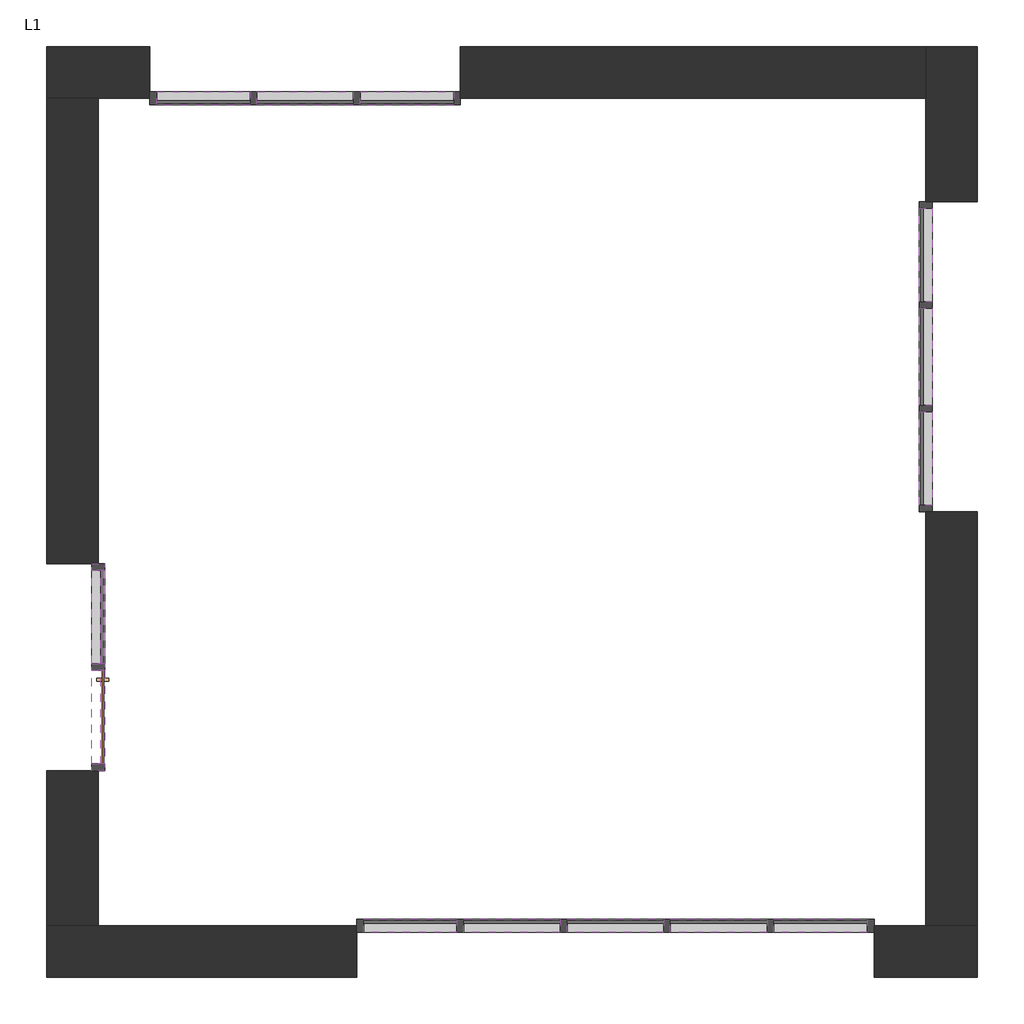
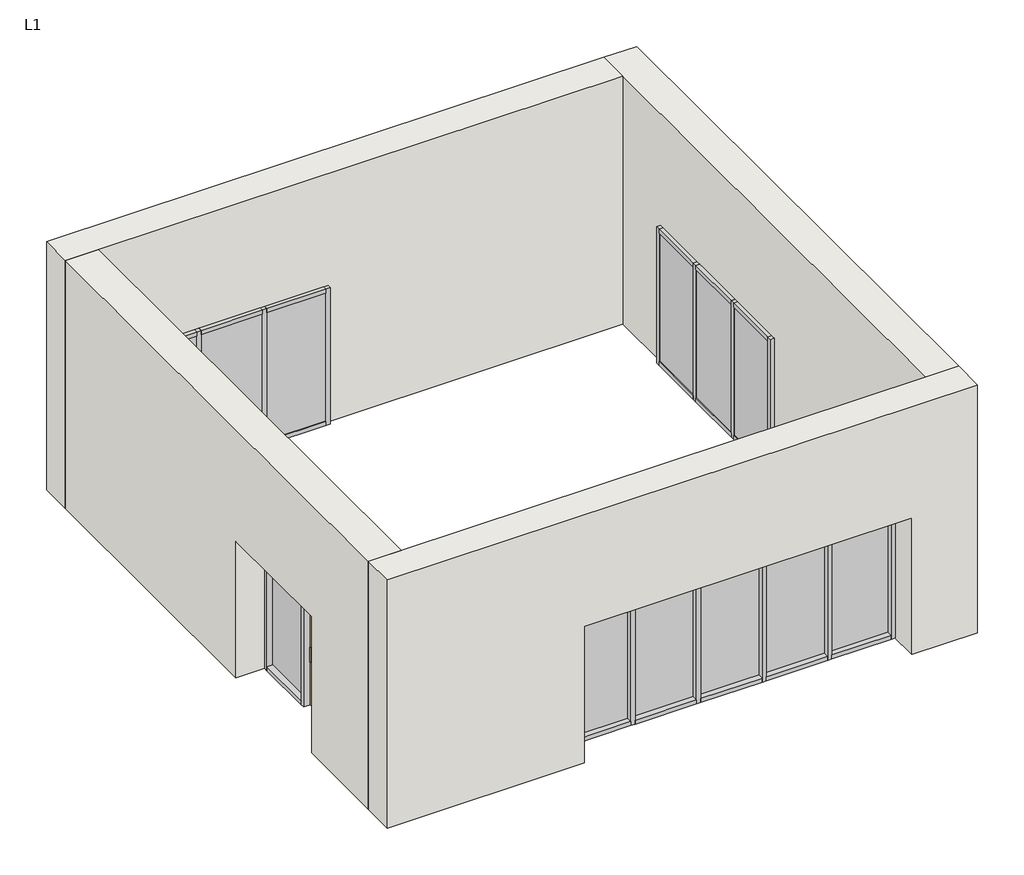
# One storey: 47 members, 14 plates, 4 walls, 1 door.
"""IFC4 building model written with IfcOpenShell, lengths in millimetres."""

import ifcopenshell
import ifcopenshell.guid

model = None  # the IFC model being written
_history = None  # IfcOwnerHistory: only IFC2X3 demands one
_inside = {}  # id of a spatial element -> (the spatial element, [elements in it])
_under = {}  # id of a project, library or spatial element -> (it, [spatial elements below it])
_declared = {}  # id of a project -> (the project, [libraries it declares])
_typed = {}  # id of a type object -> (the type object, [elements of that type])
_made_of = {}  # id of a material, layer set ... -> (it, [elements and type objects made of it])


def new_model(schema):
    """Start an empty IFC model of exactly this schema.

    Asked for "IFC4X3", IfcOpenShell would pick the latest addendum, in which some entities
    have other attributes; the version numbers below select the first issue.
    IFC2X3 requires an IfcOwnerHistory on every rooted entity: one is made here for all.
    """
    global model, _history
    if schema == "IFC4X3":
        model = ifcopenshell.file(schema_version=(4, 3, 0, 0))
    else:
        model = ifcopenshell.file(schema=schema)
    _inside.clear()
    _under.clear()
    _declared.clear()
    _typed.clear()
    _made_of.clear()
    _history = None
    if model.schema == "IFC2X3":
        org = make("IfcOrganization", Name="unknown")
        user = make(
            "IfcPersonAndOrganization",
            ThePerson=make("IfcPerson", FamilyName="unknown"),
            TheOrganization=org,
        )
        app = make(
            "IfcApplication",
            ApplicationDeveloper=org,
            Version="unknown",
            ApplicationFullName="unknown",
            ApplicationIdentifier="unknown",
        )
        _history = make(
            "IfcOwnerHistory",
            OwningUser=user,
            OwningApplication=app,
            ChangeAction="ADDED",
            CreationDate=0,
        )
    return model


def make(cls, **values):
    """One entity of the class cls with the attributes given. An attribute that is None is left unset."""
    return model.create_entity(
        cls, **{name: value for name, value in values.items() if value is not None}
    )


def rooted(cls, **values):
    """An entity with a GlobalId (a new one), such as an element, a storey or a relation."""
    return make(cls, GlobalId=ifcopenshell.guid.new(), OwnerHistory=_history, **values)


def si_unit(unit_type, name, prefix=None):
    """IfcSIUnit, for example si_unit("LENGTHUNIT", "METRE", prefix="MILLI")."""
    return make("IfcSIUnit", UnitType=unit_type, Prefix=prefix, Name=name)


def assignment(units):
    """IfcUnitAssignment: the units of a project."""
    return None if units is None else make("IfcUnitAssignment", Units=units)


def point(xyz):
    """IfcCartesianPoint."""
    return None if xyz is None else make("IfcCartesianPoint", Coordinates=xyz)


def direction(xyz):
    """IfcDirection."""
    return None if xyz is None else make("IfcDirection", DirectionRatios=xyz)


def frame(location, z_axis=None, x_axis=None):
    """IfcAxis2Placement3D, a coordinate frame: its origin and axes. An axis left out is left unset."""
    return make(
        "IfcAxis2Placement3D",
        Location=point(location),
        Axis=direction(z_axis),
        RefDirection=direction(x_axis),
    )


def origin():
    """The frame at (0, 0, 0) with its axes left unset."""
    return frame((0.0, 0.0, 0.0))


def origin_with_axes():
    """The frame at (0, 0, 0) with the z axis (0, 0, 1) and the x axis (1, 0, 0) written out."""
    return frame((0.0, 0.0, 0.0), z_axis=(0.0, 0.0, 1.0), x_axis=(1.0, 0.0, 0.0))


def place(relative_to, where):
    """IfcLocalPlacement: puts the frame where relative to a parent placement (None: the world)."""
    return make(
        "IfcLocalPlacement", PlacementRelTo=relative_to, RelativePlacement=where
    )


def context(
    kind, dimensions, precision=None, world=None, true_north=None, identifier=None
):
    """IfcGeometricRepresentationContext, for example the 3D "Model" context."""
    return make(
        "IfcGeometricRepresentationContext",
        ContextIdentifier=identifier,
        ContextType=kind,
        CoordinateSpaceDimension=dimensions,
        Precision=precision,
        WorldCoordinateSystem=world,
        TrueNorth=true_north,
    )


def project(units=None, contexts=None):
    """IfcProject with its units and contexts."""
    return rooted(
        "IfcProject",
        Name="project",
        RepresentationContexts=contexts,
        UnitsInContext=assignment(units),
    )


def spatial(cls, under=None, at=None, **own):
    """A site, building, storey or space (cls), placed at a placement, below another one or the project."""
    s = rooted(cls, ObjectPlacement=at, **own)
    if under is not None:
        _under.setdefault(under.id(), (under, []))[1].append(s)
    return s


def polyline(points):
    """IfcPolyline through the points."""
    return make("IfcPolyline", Points=[point(p) for p in points])


def outline(outer, holes=None, kind="AREA"):
    """IfcArbitraryClosedProfileDef: a profile drawn as a closed curve; with holes, ...WithVoids."""
    if holes is None:
        return make("IfcArbitraryClosedProfileDef", ProfileType=kind, OuterCurve=outer)
    return make(
        "IfcArbitraryProfileDefWithVoids",
        ProfileType=kind,
        OuterCurve=outer,
        InnerCurves=holes,
    )


def extrude(swept, where, along, depth):
    """IfcExtrudedAreaSolid: the profile swept, set in the frame where, extruded along a direction by depth."""
    return make(
        "IfcExtrudedAreaSolid",
        SweptArea=swept,
        Position=where,
        ExtrudedDirection=direction(along),
        Depth=depth,
    )


def faces_of(points, faces, orient=None, outer=None):
    """IfcFace entities. A face is a list of loops; a loop is a list of indices into points, from 0.

    orient and outer hold one flag for each loop. By default every Orientation is true, the
    first loop of a face is its IfcFaceOuterBound and the others are IfcFaceBound.
    """
    made = []
    for i, loops in enumerate(faces):
        bounds = []
        for j, loop in enumerate(loops):
            is_outer = j == 0 if outer is None else outer[i][j]
            bounds.append(
                make(
                    "IfcFaceOuterBound" if is_outer else "IfcFaceBound",
                    Bound=make("IfcPolyLoop", Polygon=[points[k] for k in loop]),
                    Orientation=True if orient is None else orient[i][j],
                )
            )
        made.append(make("IfcFace", Bounds=bounds))
    return made


def faceted_brep(points, faces, orient=None, outer=None, voids=None):
    """IfcFacetedBrep: a solid bounded by flat faces; with voids (closed shells), ...WithVoids."""
    shared = [point(p) for p in points]
    hull = make("IfcClosedShell", CfsFaces=faces_of(shared, faces, orient, outer))
    if voids is None:
        return make("IfcFacetedBrep", Outer=hull)
    return make(
        "IfcFacetedBrepWithVoids",
        Outer=hull,
        Voids=[
            make(cls, CfsFaces=faces_of(shared, fs, o, b)) for cls, fs, o, b in voids
        ],
    )


def shape(context_of_items, identifier, shape_type, items):
    """IfcShapeRepresentation: the items that make up one representation, for example the "Body"."""
    return make(
        "IfcShapeRepresentation",
        ContextOfItems=context_of_items,
        RepresentationIdentifier=identifier,
        RepresentationType=shape_type,
        Items=items,
    )


def source(mapping_origin, context_of_items, identifier, shape_type, items):
    """IfcRepresentationMap: a shape defined once, which mapped items show again and again."""
    return make(
        "IfcRepresentationMap",
        MappingOrigin=mapping_origin,
        MappedRepresentation=shape(context_of_items, identifier, shape_type, items),
    )


def transform(
    local_origin,
    x_axis=None,
    y_axis=None,
    z_axis=None,
    scale=None,
    scale2=None,
    scale3=None,
    uniform=True,
):
    """IfcCartesianTransformationOperator3D, or its non-uniform kind. x_axis, y_axis, z_axis: its Axis1, 2, 3."""
    if uniform:
        return make(
            "IfcCartesianTransformationOperator3D",
            Axis1=direction(x_axis),
            Axis2=direction(y_axis),
            LocalOrigin=point(local_origin),
            Scale=scale,
            Axis3=direction(z_axis),
        )
    return make(
        "IfcCartesianTransformationOperator3DnonUniform",
        Axis1=direction(x_axis),
        Axis2=direction(y_axis),
        LocalOrigin=point(local_origin),
        Scale=scale,
        Axis3=direction(z_axis),
        Scale2=scale2,
        Scale3=scale3,
    )


def mapped(mapping_source, mapping_target):
    """IfcMappedItem: shows the shape of a source again, moved by a transform."""
    return make(
        "IfcMappedItem", MappingSource=mapping_source, MappingTarget=mapping_target
    )


def made_of(thing, what):
    """Note that an element or type object is made of a material, layer set ...; save() writes the relation."""
    if what is not None:
        _made_of.setdefault(what.id(), (what, []))[1].append(thing)
    return thing


def element(
    cls,
    number,
    at=None,
    inside=None,
    cuts=None,
    type_object=None,
    material=None,
    context=None,
    identifier="Body",
    shape_type=None,
    held_by="IfcProductDefinitionShape",
    body=None,
    shapes=None,
    **own,
):
    """One element of the class cls, such as IfcWall. Its Tag is "e" and its number.

    at: its placement. inside: the storey or other place that contains it. cuts: it is an
    opening in that element (IfcRelVoidsElement). A single representation is given by context,
    identifier, shape_type and body (its items); several are given by shapes. held_by: the class
    of the entity that holds the representations. save() writes the other relations.
    """
    e = rooted(cls, Tag="e%d" % number, ObjectPlacement=at, **own)
    if body is not None:
        shapes = [shape(context, identifier, shape_type, body)]
    if shapes is not None:
        e.Representation = make(held_by, Representations=shapes)
    if inside is not None:
        _inside.setdefault(inside.id(), (inside, []))[1].append(e)
    if cuts is not None:
        rooted(
            "IfcRelVoidsElement", RelatingBuildingElement=cuts, RelatedOpeningElement=e
        )
    if type_object is not None:
        _typed.setdefault(type_object.id(), (type_object, []))[1].append(e)
    return made_of(e, material)


def aggregate(whole, parts):
    """IfcRelAggregates: a whole, such as a stair, and the parts it consists of."""
    return rooted("IfcRelAggregates", RelatingObject=whole, RelatedObjects=parts)


def save(model, path):
    """Write the relations noted so far, then the file.

    IfcRelAggregates (storeys below a building ...), IfcRelContainedInSpatialStructure (elements
    in a storey), IfcRelDefinesByType, IfcRelAssociatesMaterial and IfcRelDeclares: one each for
    every whole, place, type object, material and project.
    """
    for whole, parts in _under.values():
        aggregate(whole, parts)
    for where, things in _inside.values():
        rooted(
            "IfcRelContainedInSpatialStructure",
            RelatedElements=things,
            RelatingStructure=where,
        )
    for kind, things in _typed.values():
        rooted("IfcRelDefinesByType", RelatedObjects=things, RelatingType=kind)
    for what, things in _made_of.values():
        rooted("IfcRelAssociatesMaterial", RelatedObjects=things, RelatingMaterial=what)
    for by, libraries in _declared.values():
        rooted("IfcRelDeclares", RelatingContext=by, RelatedDefinitions=libraries)
    model.write(path)


def m_door_curtain_wall_single_glass_m_door_curtain_wall_single_b3f25844(model_context):
    return source(origin(), model_context, "Body", "SweptSolid", [
        extrude(outline(polyline([(451.2499998, 50.8), (451.2499998, 38.1), (-451.2499998, 38.1), (-451.2499998, 50.8), (451.2499998, 50.8)])), origin_with_axes(), (0.0, 0.0, 1.0), 1967.5),
        extrude(outline(polyline([(-375.0499998, 101.6), (-349.6499998, 101.6), (-349.6499998, 50.8), (-375.0499998, 50.8), (-375.0499998, 101.6)])), frame((0.0, 0.0, 762.0), z_axis=(0.0, 0.0, 1.0), x_axis=(1.0, 0.0, 0.0)), (0.0, 0.0, 1.0), 228.6),
        extrude(outline(polyline([(-349.6499998, -12.7), (-375.0499998, -12.7), (-375.0499998, 38.1), (-349.6499998, 38.1), (-349.6499998, -12.7)])), frame((0.0, 0.0, 762.0), z_axis=(0.0, 0.0, 1.0), x_axis=(1.0, 0.0, 0.0)), (0.0, 0.0, 1.0), 228.6),
    ])


def rectangular_mullion_65_x_125mm_rectangular_3ebb1efe(model_context):
    return source(origin(), model_context, "Body", "SweptSolid", [
        extrude(outline(polyline([(32.5, 62.5), (32.5, -62.5), (-32.5, -62.5), (-32.5, 62.5), (32.5, 62.5)])), frame((0.0, 0.0, -2200.0), z_axis=(0.0, 0.0, 1.0), x_axis=(1.0, 0.0, 0.0)), (0.0, 0.0, 1.0), 2200.0),
    ])


def rectangular_mullion_65_x_125mm_rectangular_02dc2359(model_context):
    return source(origin(), model_context, "Body", "SweptSolid", [
        extrude(outline(polyline([(0.0, 62.5), (0.0, -62.5), (-65.0, -62.5), (-65.0, 62.5), (0.0, 62.5)])), frame((0.0, 0.0, -2200.0), z_axis=(0.0, 0.0, 1.0), x_axis=(1.0, 0.0, 0.0)), (0.0, 0.0, 1.0), 2200.0),
    ])


def rectangular_mullion_65_x_125mm_rectangular_9a77bebc(model_context):
    return source(origin(), model_context, "Body", "SweptSolid", [
        extrude(outline(polyline([(0.0, 62.5), (0.0, -62.5), (-65.0, -62.5), (-65.0, 62.5), (0.0, 62.5)])), frame((0.0, 0.0, -902.5000003), z_axis=(0.0, 0.0, 1.0), x_axis=(1.0, 0.0, 0.0)), (0.0, 0.0, 1.0), 902.5000003),
    ])


def rectangular_mullion_65_x_125mm_rectangular_1b57746c(model_context):
    return source(origin(), model_context, "Body", "SweptSolid", [
        extrude(outline(polyline([(0.0, 62.5), (0.0, -62.5), (-65.0, -62.5), (-65.0, 62.5), (0.0, 62.5)])), frame((0.0, 0.0, -935.0), z_axis=(0.0, 0.0, 1.0), x_axis=(1.0, 0.0, 0.0)), (0.0, 0.0, 1.0), 935.0),
    ])


def rectangular_mullion_65_x_125mm_rectangular_ad388592(model_context):
    return source(origin(), model_context, "Body", "SweptSolid", [
        extrude(outline(polyline([(32.5, 62.5), (32.5, -62.5), (-32.5, -62.5), (-32.5, 62.5), (32.5, 62.5)])), frame((0.0, 0.0, -902.5000003), z_axis=(0.0, 0.0, 1.0), x_axis=(1.0, 0.0, 0.0)), (0.0, 0.0, 1.0), 902.5000003),
    ])


def rectangular_mullion_65_x_125mm_rectangular_470365d3(model_context):
    return source(origin(), model_context, "Body", "SweptSolid", [
        extrude(outline(polyline([(32.5, 62.5), (32.5, -62.5), (-32.5, -62.5), (-32.5, 62.5), (32.5, 62.5)])), frame((0.0, 0.0, -200.0), z_axis=(0.0, 0.0, 1.0), x_axis=(1.0, 0.0, 0.0)), (0.0, 0.0, 1.0), 200.0),
    ])


def rectangular_mullion_65_x_125mm_rectangular_dd0f1ba9(model_context):
    return source(origin(), model_context, "Body", "SweptSolid", [
        extrude(outline(polyline([(0.0, 62.5), (0.0, -62.5), (-65.0, -62.5), (-65.0, 62.5), (0.0, 62.5)])), frame((0.0, 0.0, -200.0), z_axis=(0.0, 0.0, 1.0), x_axis=(1.0, 0.0, 0.0)), (0.0, 0.0, 1.0), 200.0),
    ])


def rectangular_mullion_65_x_125mm_rectangular_b62c991d(model_context):
    return source(origin(), model_context, "Body", "SweptSolid", [
        extrude(outline(polyline([(32.5, 62.5), (32.5, -62.5), (-32.5, -62.5), (-32.5, 62.5), (32.5, 62.5)])), frame((0.0, 0.0, -2000.0), z_axis=(0.0, 0.0, 1.0), x_axis=(1.0, 0.0, 0.0)), (0.0, 0.0, 1.0), 2000.0),
    ])


def rectangular_mullion_65_x_125mm_rectangular_d57ab73f(model_context):
    return source(origin(), model_context, "Body", "SweptSolid", [
        extrude(outline(polyline([(0.0, 62.5), (0.0, -62.5), (-65.0, -62.5), (-65.0, 62.5), (0.0, 62.5)])), frame((0.0, 0.0, -2000.0), z_axis=(0.0, 0.0, 1.0), x_axis=(1.0, 0.0, 0.0)), (0.0, 0.0, 1.0), 2000.0),
    ])


def system_panel_glazed_3f8cfcef(model_context):
    return source(origin(), model_context, "Body", "SweptSolid", [
        extrude(outline(polyline([(451.2500002, 24.5), (-451.2500002, 24.5), (-451.2500002, 49.5), (451.2500002, 49.5), (451.2500002, 24.5)])), origin_with_axes(), (0.0, 0.0, 1.0), 2070.0),
    ])


def system_panel_glazed_4c7b465e(model_context):
    return source(origin(), model_context, "Body", "SweptSolid", [
        extrude(outline(polyline([(467.5, 24.5), (-467.5, 24.5), (-467.5, 49.5), (467.5, 49.5), (467.5, 24.5)])), origin_with_axes(), (0.0, 0.0, 1.0), 2070.0),
    ])


def system_panel_glazed_7330a8e7(model_context):
    return source(origin(), model_context, "Body", "SweptSolid", [
        extrude(outline(polyline([(451.2500002, 24.5), (-451.2500002, 24.5), (-451.2500002, 49.5), (451.2500002, 49.5), (451.2500002, 24.5)])), origin_with_axes(), (0.0, 0.0, 1.0), 102.5),
    ])


def system_panel_glazed_53f32d20(model_context):
    return source(origin(), model_context, "Body", "SweptSolid", [
        extrude(outline(polyline([(451.2500002, 24.5), (-451.2500002, 24.5), (-451.2500002, 49.5), (451.2500002, 49.5), (451.2500002, 24.5)])), origin_with_axes(), (0.0, 0.0, 1.0), 1902.5),
    ])


model = new_model("IFC4")

# Units and contexts
model_context = context("Model", 3, world=origin())
ifc_project = project(units=[si_unit("LENGTHUNIT", "METRE", prefix="MILLI")], contexts=[model_context])

# Site, building, storey
site = spatial("IfcSite", under=ifc_project)
building = spatial("IfcBuilding", under=site)
storey = spatial("IfcBuildingStorey", under=building, Name="L1", Elevation=0.0)

# Door
placement = place(None, origin())
m_door_curtain_wall_single_glass_m_door_curtain_wall_single_shape = m_door_curtain_wall_single_glass_m_door_curtain_wall_single_b3f25844(model_context)
element("IfcDoor", 1, ObjectType="M_Door-Curtain-Wall-Single-Glass : M_Door-Curtain-Wall-Single-Glass", at=placement, inside=storey, context=model_context, shape_type="MappedRepresentation", body=[
    mapped(m_door_curtain_wall_single_glass_m_door_curtain_wall_single_shape, transform((500.000016, 1516.2441438, 0.0), x_axis=(0.0, -1.0, 0.0), y_axis=(1.0, 0.0, 0.0), z_axis=(0.0, 0.0, 1.0))),
])

# Members
rectangular_mullion_65_x_125mm_rectangular_shape = rectangular_mullion_65_x_125mm_rectangular_3ebb1efe(model_context)
element("IfcMember", 2, ObjectType="Rectangular Mullion : 65 x 125mm rectangular", at=placement, inside=storey, context=model_context, shape_type="MappedRepresentation", body=[
    mapped(rectangular_mullion_65_x_125mm_rectangular_shape, transform((4000.0000163, -500.005856, 0.0), x_axis=(1.0, 0.0, 0.0), y_axis=(0.0, -1.0, 0.0), z_axis=(0.0, 0.0, -1.0))),
])
element("IfcMember", 3, ObjectType="Rectangular Mullion : 65 x 125mm rectangular", at=placement, inside=storey, context=model_context, shape_type="MappedRepresentation", body=[
    mapped(rectangular_mullion_65_x_125mm_rectangular_shape, transform((5000.0000163, -500.005856, 0.0), x_axis=(1.0, 0.0, 0.0), y_axis=(0.0, -1.0, 0.0), z_axis=(0.0, 0.0, -1.0))),
])
element("IfcMember", 4, ObjectType="Rectangular Mullion : 65 x 125mm rectangular", at=placement, inside=storey, context=model_context, shape_type="MappedRepresentation", body=[
    mapped(rectangular_mullion_65_x_125mm_rectangular_shape, transform((6000.0000163, -500.005856, 0.0), x_axis=(1.0, 0.0, 0.0), y_axis=(0.0, -1.0, 0.0), z_axis=(0.0, 0.0, -1.0))),
])
element("IfcMember", 5, ObjectType="Rectangular Mullion : 65 x 125mm rectangular", at=placement, inside=storey, context=model_context, shape_type="MappedRepresentation", body=[
    mapped(rectangular_mullion_65_x_125mm_rectangular_shape, transform((7000.0000163, -500.005856, 0.0), x_axis=(1.0, 0.0, 0.0), y_axis=(0.0, -1.0, 0.0), z_axis=(0.0, 0.0, -1.0))),
])
element("IfcMember", 6, ObjectType="Rectangular Mullion : 65 x 125mm rectangular", at=placement, inside=storey, context=model_context, shape_type="MappedRepresentation", body=[
    mapped(rectangular_mullion_65_x_125mm_rectangular_shape, transform((8500.000016, 4499.9941443, 0.0), x_axis=(0.0, 1.0, 0.0), y_axis=(1.0, 0.0, 0.0), z_axis=(0.0, 0.0, -1.0))),
])
element("IfcMember", 7, ObjectType="Rectangular Mullion : 65 x 125mm rectangular", at=placement, inside=storey, context=model_context, shape_type="MappedRepresentation", body=[
    mapped(rectangular_mullion_65_x_125mm_rectangular_shape, transform((8500.000016, 5499.9941443, 0.0), x_axis=(0.0, 1.0, 0.0), y_axis=(1.0, 0.0, 0.0), z_axis=(0.0, 0.0, -1.0))),
])
element("IfcMember", 8, ObjectType="Rectangular Mullion : 65 x 125mm rectangular", at=placement, inside=storey, context=model_context, shape_type="MappedRepresentation", body=[
    mapped(rectangular_mullion_65_x_125mm_rectangular_shape, transform((3000.0000157, 7499.994144, 0.0), x_axis=(-1.0, 0.0, 0.0), y_axis=(0.0, 1.0, 0.0), z_axis=(0.0, 0.0, -1.0))),
])
element("IfcMember", 9, ObjectType="Rectangular Mullion : 65 x 125mm rectangular", at=placement, inside=storey, context=model_context, shape_type="MappedRepresentation", body=[
    mapped(rectangular_mullion_65_x_125mm_rectangular_shape, transform((2000.0000157, 7499.994144, 0.0), x_axis=(-1.0, 0.0, 0.0), y_axis=(0.0, 1.0, 0.0), z_axis=(0.0, 0.0, -1.0))),
])
rectangular_mullion_65_x_125mm_rectangular_2_shape = rectangular_mullion_65_x_125mm_rectangular_02dc2359(model_context)
element("IfcMember", 10, ObjectType="Rectangular Mullion : 65 x 125mm rectangular", at=placement, inside=storey, context=model_context, shape_type="MappedRepresentation", body=[
    mapped(rectangular_mullion_65_x_125mm_rectangular_2_shape, transform((8000.000016, -500.005856, 0.0), x_axis=(1.0, 0.0, 0.0), y_axis=(0.0, -1.0, 0.0), z_axis=(0.0, 0.0, -1.0))),
])
element("IfcMember", 11, ObjectType="Rectangular Mullion : 65 x 125mm rectangular", at=placement, inside=storey, context=model_context, shape_type="MappedRepresentation", body=[
    mapped(rectangular_mullion_65_x_125mm_rectangular_2_shape, transform((8500.000016, 6499.994144, 0.0), x_axis=(0.0, 1.0, 0.0), y_axis=(1.0, 0.0, 0.0), z_axis=(0.0, 0.0, -1.0))),
])
element("IfcMember", 12, ObjectType="Rectangular Mullion : 65 x 125mm rectangular", at=placement, inside=storey, context=model_context, shape_type="MappedRepresentation", body=[
    mapped(rectangular_mullion_65_x_125mm_rectangular_2_shape, transform((1000.000016, 7499.994144, 0.0), x_axis=(-1.0, 0.0, 0.0), y_axis=(0.0, 1.0, 0.0), z_axis=(0.0, 0.0, -1.0))),
])
element("IfcMember", 13, ObjectType="Rectangular Mullion : 65 x 125mm rectangular", at=placement, inside=storey, context=model_context, shape_type="MappedRepresentation", body=[
    mapped(rectangular_mullion_65_x_125mm_rectangular_2_shape, transform((3000.000016, -500.005856, 2200.0), x_axis=(-1.0, 0.0, 0.0), y_axis=(0.0, -1.0, 0.0), z_axis=(0.0, 0.0, 1.0))),
])
element("IfcMember", 14, ObjectType="Rectangular Mullion : 65 x 125mm rectangular", at=placement, inside=storey, context=model_context, shape_type="MappedRepresentation", body=[
    mapped(rectangular_mullion_65_x_125mm_rectangular_2_shape, transform((8500.000016, 3499.994144, 2200.0), x_axis=(0.0, -1.0, 0.0), y_axis=(1.0, 0.0, 0.0), z_axis=(0.0, 0.0, 1.0))),
])
element("IfcMember", 15, ObjectType="Rectangular Mullion : 65 x 125mm rectangular", at=placement, inside=storey, context=model_context, shape_type="MappedRepresentation", body=[
    mapped(rectangular_mullion_65_x_125mm_rectangular_2_shape, transform((4000.000016, 7499.994144, 2200.0), x_axis=(1.0, 0.0, 0.0), y_axis=(0.0, 1.0, 0.0), z_axis=(0.0, 0.0, 1.0))),
])
rectangular_mullion_65_x_125mm_rectangular_3_shape = rectangular_mullion_65_x_125mm_rectangular_9a77bebc(model_context)
element("IfcMember", 16, ObjectType="Rectangular Mullion : 65 x 125mm rectangular", at=placement, inside=storey, context=model_context, shape_type="MappedRepresentation", body=[
    mapped(rectangular_mullion_65_x_125mm_rectangular_3_shape, transform((7935.000016, -500.005856, 2200.0), x_axis=(0.0, 0.0, 1.0), y_axis=(0.0, -1.0, 0.0), z_axis=(1.0, 0.0, 0.0))),
])
element("IfcMember", 17, ObjectType="Rectangular Mullion : 65 x 125mm rectangular", at=placement, inside=storey, context=model_context, shape_type="MappedRepresentation", body=[
    mapped(rectangular_mullion_65_x_125mm_rectangular_3_shape, transform((3967.5000163, -500.005856, 2200.0), x_axis=(0.0, 0.0, 1.0), y_axis=(0.0, -1.0, 0.0), z_axis=(1.0, 0.0, 0.0))),
])
element("IfcMember", 18, ObjectType="Rectangular Mullion : 65 x 125mm rectangular", at=placement, inside=storey, context=model_context, shape_type="MappedRepresentation", body=[
    mapped(rectangular_mullion_65_x_125mm_rectangular_3_shape, transform((8500.000016, 6434.994144, 2200.0), x_axis=(0.0, 0.0, 1.0), y_axis=(1.0, 0.0, 0.0), z_axis=(0.0, 1.0, 0.0))),
])
element("IfcMember", 19, ObjectType="Rectangular Mullion : 65 x 125mm rectangular", at=placement, inside=storey, context=model_context, shape_type="MappedRepresentation", body=[
    mapped(rectangular_mullion_65_x_125mm_rectangular_3_shape, transform((8500.000016, 4467.4941443, 2200.0), x_axis=(0.0, 0.0, 1.0), y_axis=(1.0, 0.0, 0.0), z_axis=(0.0, 1.0, 0.0))),
])
element("IfcMember", 20, ObjectType="Rectangular Mullion : 65 x 125mm rectangular", at=placement, inside=storey, context=model_context, shape_type="MappedRepresentation", body=[
    mapped(rectangular_mullion_65_x_125mm_rectangular_3_shape, transform((1065.000016, 7499.994144, 2200.0), x_axis=(0.0, 0.0, 1.0), y_axis=(0.0, 1.0, 0.0), z_axis=(-1.0, 0.0, 0.0))),
])
element("IfcMember", 21, ObjectType="Rectangular Mullion : 65 x 125mm rectangular", at=placement, inside=storey, context=model_context, shape_type="MappedRepresentation", body=[
    mapped(rectangular_mullion_65_x_125mm_rectangular_3_shape, transform((3032.5000157, 7499.994144, 2200.0), x_axis=(0.0, 0.0, 1.0), y_axis=(0.0, 1.0, 0.0), z_axis=(-1.0, 0.0, 0.0))),
])
element("IfcMember", 22, ObjectType="Rectangular Mullion : 65 x 125mm rectangular", at=placement, inside=storey, context=model_context, shape_type="MappedRepresentation", body=[
    mapped(rectangular_mullion_65_x_125mm_rectangular_3_shape, transform((500.000016, 1064.994144, 2200.0), x_axis=(0.0, 0.0, 1.0), y_axis=(-1.0, 0.0, 0.0), z_axis=(0.0, -1.0, 0.0))),
])
element("IfcMember", 23, ObjectType="Rectangular Mullion : 65 x 125mm rectangular", at=placement, inside=storey, context=model_context, shape_type="MappedRepresentation", body=[
    mapped(rectangular_mullion_65_x_125mm_rectangular_3_shape, transform((500.000016, 2032.4941437, 2200.0), x_axis=(0.0, 0.0, 1.0), y_axis=(-1.0, 0.0, 0.0), z_axis=(0.0, -1.0, 0.0))),
])
rectangular_mullion_65_x_125mm_rectangular_4_shape = rectangular_mullion_65_x_125mm_rectangular_1b57746c(model_context)
element("IfcMember", 24, ObjectType="Rectangular Mullion : 65 x 125mm rectangular", at=placement, inside=storey, context=model_context, shape_type="MappedRepresentation", body=[
    mapped(rectangular_mullion_65_x_125mm_rectangular_4_shape, transform((4967.5000163, -500.005856, 2200.0), x_axis=(0.0, 0.0, 1.0), y_axis=(0.0, -1.0, 0.0), z_axis=(1.0, 0.0, 0.0))),
])
element("IfcMember", 25, ObjectType="Rectangular Mullion : 65 x 125mm rectangular", at=placement, inside=storey, context=model_context, shape_type="MappedRepresentation", body=[
    mapped(rectangular_mullion_65_x_125mm_rectangular_4_shape, transform((5967.5000163, -500.005856, 2200.0), x_axis=(0.0, 0.0, 1.0), y_axis=(0.0, -1.0, 0.0), z_axis=(1.0, 0.0, 0.0))),
])
element("IfcMember", 26, ObjectType="Rectangular Mullion : 65 x 125mm rectangular", at=placement, inside=storey, context=model_context, shape_type="MappedRepresentation", body=[
    mapped(rectangular_mullion_65_x_125mm_rectangular_4_shape, transform((6967.5000163, -500.005856, 2200.0), x_axis=(0.0, 0.0, 1.0), y_axis=(0.0, -1.0, 0.0), z_axis=(1.0, 0.0, 0.0))),
])
element("IfcMember", 27, ObjectType="Rectangular Mullion : 65 x 125mm rectangular", at=placement, inside=storey, context=model_context, shape_type="MappedRepresentation", body=[
    mapped(rectangular_mullion_65_x_125mm_rectangular_4_shape, transform((8500.000016, 5467.4941443, 2200.0), x_axis=(0.0, 0.0, 1.0), y_axis=(1.0, 0.0, 0.0), z_axis=(0.0, 1.0, 0.0))),
])
element("IfcMember", 28, ObjectType="Rectangular Mullion : 65 x 125mm rectangular", at=placement, inside=storey, context=model_context, shape_type="MappedRepresentation", body=[
    mapped(rectangular_mullion_65_x_125mm_rectangular_4_shape, transform((2032.5000157, 7499.994144, 2200.0), x_axis=(0.0, 0.0, 1.0), y_axis=(0.0, 1.0, 0.0), z_axis=(-1.0, 0.0, 0.0))),
])
element("IfcMember", 29, ObjectType="Rectangular Mullion : 65 x 125mm rectangular", at=placement, inside=storey, context=model_context, shape_type="MappedRepresentation", body=[
    mapped(rectangular_mullion_65_x_125mm_rectangular_3_shape, transform((3065.000016, -500.005856, 0.0), x_axis=(0.0, 0.0, -1.0), y_axis=(0.0, -1.0, 0.0), z_axis=(-1.0, 0.0, 0.0))),
])
element("IfcMember", 30, ObjectType="Rectangular Mullion : 65 x 125mm rectangular", at=placement, inside=storey, context=model_context, shape_type="MappedRepresentation", body=[
    mapped(rectangular_mullion_65_x_125mm_rectangular_3_shape, transform((7032.5000163, -500.005856, 0.0), x_axis=(0.0, 0.0, -1.0), y_axis=(0.0, -1.0, 0.0), z_axis=(-1.0, 0.0, 0.0))),
])
element("IfcMember", 31, ObjectType="Rectangular Mullion : 65 x 125mm rectangular", at=placement, inside=storey, context=model_context, shape_type="MappedRepresentation", body=[
    mapped(rectangular_mullion_65_x_125mm_rectangular_3_shape, transform((8500.000016, 3564.994144, 0.0), x_axis=(0.0, 0.0, -1.0), y_axis=(1.0, 0.0, 0.0), z_axis=(0.0, -1.0, 0.0))),
])
element("IfcMember", 32, ObjectType="Rectangular Mullion : 65 x 125mm rectangular", at=placement, inside=storey, context=model_context, shape_type="MappedRepresentation", body=[
    mapped(rectangular_mullion_65_x_125mm_rectangular_3_shape, transform((8500.000016, 5532.4941443, 0.0), x_axis=(0.0, 0.0, -1.0), y_axis=(1.0, 0.0, 0.0), z_axis=(0.0, -1.0, 0.0))),
])
element("IfcMember", 33, ObjectType="Rectangular Mullion : 65 x 125mm rectangular", at=placement, inside=storey, context=model_context, shape_type="MappedRepresentation", body=[
    mapped(rectangular_mullion_65_x_125mm_rectangular_3_shape, transform((3935.000016, 7499.994144, 0.0), x_axis=(0.0, 0.0, -1.0), y_axis=(0.0, 1.0, 0.0), z_axis=(1.0, 0.0, 0.0))),
])
element("IfcMember", 34, ObjectType="Rectangular Mullion : 65 x 125mm rectangular", at=placement, inside=storey, context=model_context, shape_type="MappedRepresentation", body=[
    mapped(rectangular_mullion_65_x_125mm_rectangular_3_shape, transform((1967.5000157, 7499.994144, 0.0), x_axis=(0.0, 0.0, -1.0), y_axis=(0.0, 1.0, 0.0), z_axis=(1.0, 0.0, 0.0))),
])
element("IfcMember", 35, ObjectType="Rectangular Mullion : 65 x 125mm rectangular", at=placement, inside=storey, context=model_context, shape_type="MappedRepresentation", body=[
    mapped(rectangular_mullion_65_x_125mm_rectangular_3_shape, transform((500.000016, 2934.994144, 0.0), x_axis=(0.0, 0.0, -1.0), y_axis=(-1.0, 0.0, 0.0), z_axis=(0.0, 1.0, 0.0))),
])
element("IfcMember", 36, ObjectType="Rectangular Mullion : 65 x 125mm rectangular", at=placement, inside=storey, context=model_context, shape_type="MappedRepresentation", body=[
    mapped(rectangular_mullion_65_x_125mm_rectangular_4_shape, transform((4032.5000163, -500.005856, 0.0), x_axis=(0.0, 0.0, -1.0), y_axis=(0.0, -1.0, 0.0), z_axis=(-1.0, 0.0, 0.0))),
])
element("IfcMember", 37, ObjectType="Rectangular Mullion : 65 x 125mm rectangular", at=placement, inside=storey, context=model_context, shape_type="MappedRepresentation", body=[
    mapped(rectangular_mullion_65_x_125mm_rectangular_4_shape, transform((5032.5000163, -500.005856, 0.0), x_axis=(0.0, 0.0, -1.0), y_axis=(0.0, -1.0, 0.0), z_axis=(-1.0, 0.0, 0.0))),
])
element("IfcMember", 38, ObjectType="Rectangular Mullion : 65 x 125mm rectangular", at=placement, inside=storey, context=model_context, shape_type="MappedRepresentation", body=[
    mapped(rectangular_mullion_65_x_125mm_rectangular_4_shape, transform((6032.5000163, -500.005856, 0.0), x_axis=(0.0, 0.0, -1.0), y_axis=(0.0, -1.0, 0.0), z_axis=(-1.0, 0.0, 0.0))),
])
element("IfcMember", 39, ObjectType="Rectangular Mullion : 65 x 125mm rectangular", at=placement, inside=storey, context=model_context, shape_type="MappedRepresentation", body=[
    mapped(rectangular_mullion_65_x_125mm_rectangular_4_shape, transform((8500.000016, 4532.4941443, 0.0), x_axis=(0.0, 0.0, -1.0), y_axis=(1.0, 0.0, 0.0), z_axis=(0.0, -1.0, 0.0))),
])
element("IfcMember", 40, ObjectType="Rectangular Mullion : 65 x 125mm rectangular", at=placement, inside=storey, context=model_context, shape_type="MappedRepresentation", body=[
    mapped(rectangular_mullion_65_x_125mm_rectangular_4_shape, transform((2967.5000157, 7499.994144, 0.0), x_axis=(0.0, 0.0, -1.0), y_axis=(0.0, 1.0, 0.0), z_axis=(1.0, 0.0, 0.0))),
])
rectangular_mullion_65_x_125mm_rectangular_5_shape = rectangular_mullion_65_x_125mm_rectangular_ad388592(model_context)
element("IfcMember", 41, ObjectType="Rectangular Mullion : 65 x 125mm rectangular", at=placement, inside=storey, context=model_context, shape_type="MappedRepresentation", body=[
    mapped(rectangular_mullion_65_x_125mm_rectangular_5_shape, transform((500.000016, 2032.4941437, 2000.0), x_axis=(0.0, 0.0, 1.0), y_axis=(-1.0, 0.0, 0.0), z_axis=(0.0, -1.0, 0.0))),
])
element("IfcMember", 42, ObjectType="Rectangular Mullion : 65 x 125mm rectangular", at=placement, inside=storey, context=model_context, shape_type="MappedRepresentation", body=[
    mapped(rectangular_mullion_65_x_125mm_rectangular_5_shape, transform((500.000016, 1064.994144, 2000.0), x_axis=(0.0, 0.0, 1.0), y_axis=(-1.0, 0.0, 0.0), z_axis=(0.0, -1.0, 0.0))),
])
rectangular_mullion_65_x_125mm_rectangular_6_shape = rectangular_mullion_65_x_125mm_rectangular_470365d3(model_context)
element("IfcMember", 43, ObjectType="Rectangular Mullion : 65 x 125mm rectangular", at=placement, inside=storey, context=model_context, shape_type="MappedRepresentation", body=[
    mapped(rectangular_mullion_65_x_125mm_rectangular_6_shape, transform((500.000016, 1999.9941437, 2000.0), x_axis=(0.0, -1.0, 0.0), y_axis=(-1.0, 0.0, 0.0), z_axis=(0.0, 0.0, -1.0))),
])
rectangular_mullion_65_x_125mm_rectangular_7_shape = rectangular_mullion_65_x_125mm_rectangular_dd0f1ba9(model_context)
element("IfcMember", 44, ObjectType="Rectangular Mullion : 65 x 125mm rectangular", at=placement, inside=storey, context=model_context, shape_type="MappedRepresentation", body=[
    mapped(rectangular_mullion_65_x_125mm_rectangular_7_shape, transform((500.000016, 999.994144, 2000.0), x_axis=(0.0, -1.0, 0.0), y_axis=(-1.0, 0.0, 0.0), z_axis=(0.0, 0.0, -1.0))),
])
element("IfcMember", 45, ObjectType="Rectangular Mullion : 65 x 125mm rectangular", at=placement, inside=storey, context=model_context, shape_type="MappedRepresentation", body=[
    mapped(rectangular_mullion_65_x_125mm_rectangular_7_shape, transform((500.000016, 2999.994144, 2200.0), x_axis=(0.0, 1.0, 0.0), y_axis=(-1.0, 0.0, 0.0), z_axis=(0.0, 0.0, 1.0))),
])
rectangular_mullion_65_x_125mm_rectangular_8_shape = rectangular_mullion_65_x_125mm_rectangular_b62c991d(model_context)
element("IfcMember", 46, ObjectType="Rectangular Mullion : 65 x 125mm rectangular", at=placement, inside=storey, context=model_context, shape_type="MappedRepresentation", body=[
    mapped(rectangular_mullion_65_x_125mm_rectangular_8_shape, transform((500.000016, 1999.9941437, 0.0), x_axis=(0.0, -1.0, 0.0), y_axis=(-1.0, 0.0, 0.0), z_axis=(0.0, 0.0, -1.0))),
])
rectangular_mullion_65_x_125mm_rectangular_9_shape = rectangular_mullion_65_x_125mm_rectangular_d57ab73f(model_context)
element("IfcMember", 47, ObjectType="Rectangular Mullion : 65 x 125mm rectangular", at=placement, inside=storey, context=model_context, shape_type="MappedRepresentation", body=[
    mapped(rectangular_mullion_65_x_125mm_rectangular_9_shape, transform((500.000016, 2999.994144, 2000.0), x_axis=(0.0, 1.0, 0.0), y_axis=(-1.0, 0.0, 0.0), z_axis=(0.0, 0.0, 1.0))),
])
element("IfcMember", 48, ObjectType="Rectangular Mullion : 65 x 125mm rectangular", at=placement, inside=storey, context=model_context, shape_type="MappedRepresentation", body=[
    mapped(rectangular_mullion_65_x_125mm_rectangular_9_shape, transform((500.000016, 999.994144, 0.0), x_axis=(0.0, -1.0, 0.0), y_axis=(-1.0, 0.0, 0.0), z_axis=(0.0, 0.0, -1.0))),
])

# Plates
system_panel_glazed_shape = system_panel_glazed_3f8cfcef(model_context)
element("IfcPlate", 49, ObjectType="System Panel : Glazed", at=placement, inside=storey, context=model_context, shape_type="MappedRepresentation", body=[
    mapped(system_panel_glazed_shape, transform((3516.2500162, -500.005856, 65.0), x_axis=(1.0, 0.0, 0.0), y_axis=(0.0, 1.0, 0.0), z_axis=(0.0, 0.0, 1.0))),
])
element("IfcPlate", 50, ObjectType="System Panel : Glazed", at=placement, inside=storey, context=model_context, shape_type="MappedRepresentation", body=[
    mapped(system_panel_glazed_shape, transform((7483.7500162, -500.005856, 65.0), x_axis=(1.0, 0.0, 0.0), y_axis=(0.0, 1.0, 0.0), z_axis=(0.0, 0.0, 1.0))),
])
element("IfcPlate", 51, ObjectType="System Panel : Glazed", at=placement, inside=storey, context=model_context, shape_type="MappedRepresentation", body=[
    mapped(system_panel_glazed_shape, transform((8500.000016, 4016.2441442, 65.0), x_axis=(0.0, 1.0, 0.0), y_axis=(-1.0, 0.0, 0.0), z_axis=(0.0, 0.0, 1.0))),
])
element("IfcPlate", 52, ObjectType="System Panel : Glazed", at=placement, inside=storey, context=model_context, shape_type="MappedRepresentation", body=[
    mapped(system_panel_glazed_shape, transform((8500.000016, 5983.7441442, 65.0), x_axis=(0.0, 1.0, 0.0), y_axis=(-1.0, 0.0, 0.0), z_axis=(0.0, 0.0, 1.0))),
])
element("IfcPlate", 53, ObjectType="System Panel : Glazed", at=placement, inside=storey, context=model_context, shape_type="MappedRepresentation", body=[
    mapped(system_panel_glazed_shape, transform((3483.7500158, 7499.994144, 65.0), x_axis=(-1.0, 0.0, 0.0), y_axis=(0.0, -1.0, 0.0), z_axis=(0.0, 0.0, 1.0))),
])
element("IfcPlate", 54, ObjectType="System Panel : Glazed", at=placement, inside=storey, context=model_context, shape_type="MappedRepresentation", body=[
    mapped(system_panel_glazed_shape, transform((1516.2500158, 7499.994144, 65.0), x_axis=(-1.0, 0.0, 0.0), y_axis=(0.0, -1.0, 0.0), z_axis=(0.0, 0.0, 1.0))),
])
system_panel_glazed_2_shape = system_panel_glazed_4c7b465e(model_context)
element("IfcPlate", 55, ObjectType="System Panel : Glazed", at=placement, inside=storey, context=model_context, shape_type="MappedRepresentation", body=[
    mapped(system_panel_glazed_2_shape, transform((4500.0000163, -500.005856, 65.0), x_axis=(1.0, 0.0, 0.0), y_axis=(0.0, 1.0, 0.0), z_axis=(0.0, 0.0, 1.0))),
])
element("IfcPlate", 56, ObjectType="System Panel : Glazed", at=placement, inside=storey, context=model_context, shape_type="MappedRepresentation", body=[
    mapped(system_panel_glazed_2_shape, transform((5500.0000163, -500.005856, 65.0), x_axis=(1.0, 0.0, 0.0), y_axis=(0.0, 1.0, 0.0), z_axis=(0.0, 0.0, 1.0))),
])
element("IfcPlate", 57, ObjectType="System Panel : Glazed", at=placement, inside=storey, context=model_context, shape_type="MappedRepresentation", body=[
    mapped(system_panel_glazed_2_shape, transform((6500.0000163, -500.005856, 65.0), x_axis=(1.0, 0.0, 0.0), y_axis=(0.0, 1.0, 0.0), z_axis=(0.0, 0.0, 1.0))),
])
element("IfcPlate", 58, ObjectType="System Panel : Glazed", at=placement, inside=storey, context=model_context, shape_type="MappedRepresentation", body=[
    mapped(system_panel_glazed_2_shape, transform((8500.000016, 4999.9941443, 65.0), x_axis=(0.0, 1.0, 0.0), y_axis=(-1.0, 0.0, 0.0), z_axis=(0.0, 0.0, 1.0))),
])
element("IfcPlate", 59, ObjectType="System Panel : Glazed", at=placement, inside=storey, context=model_context, shape_type="MappedRepresentation", body=[
    mapped(system_panel_glazed_2_shape, transform((2500.0000157, 7499.994144, 65.0), x_axis=(-1.0, 0.0, 0.0), y_axis=(0.0, -1.0, 0.0), z_axis=(0.0, 0.0, 1.0))),
])
system_panel_glazed_3_shape = system_panel_glazed_7330a8e7(model_context)
element("IfcPlate", 60, ObjectType="System Panel : Glazed", at=placement, inside=storey, context=model_context, shape_type="MappedRepresentation", body=[
    mapped(system_panel_glazed_3_shape, transform((500.000016, 2483.7441438, 2032.5), x_axis=(0.0, -1.0, 0.0), y_axis=(1.0, 0.0, 0.0), z_axis=(0.0, 0.0, 1.0))),
])
element("IfcPlate", 61, ObjectType="System Panel : Glazed", at=placement, inside=storey, context=model_context, shape_type="MappedRepresentation", body=[
    mapped(system_panel_glazed_3_shape, transform((500.000016, 1516.2441438, 2032.5), x_axis=(0.0, -1.0, 0.0), y_axis=(1.0, 0.0, 0.0), z_axis=(0.0, 0.0, 1.0))),
])
system_panel_glazed_4_shape = system_panel_glazed_53f32d20(model_context)
element("IfcPlate", 62, ObjectType="System Panel : Glazed", at=placement, inside=storey, context=model_context, shape_type="MappedRepresentation", body=[
    mapped(system_panel_glazed_4_shape, transform((500.000016, 2483.7441438, 65.0), x_axis=(0.0, -1.0, 0.0), y_axis=(1.0, 0.0, 0.0), z_axis=(0.0, 0.0, 1.0))),
])

# Walls
element("IfcWall", 63, ObjectType="MURO EXTERIOR0.60", at=placement, inside=storey, context=model_context, shape_type="Brep", body=[
    faceted_brep([(9000.000032, -1000.005872, 4000.01232), (0.0, -1000.005872, 4000.01232), (0.0, -1000.005872, 0.0), (3000.000016, -1000.005872, 0.0), (3000.000016, -1000.005872, 2200.0), (8000.000016, -1000.005872, 2200.0), (8000.000016, -1000.005872, 0.0), (9000.000032, -1000.005872, 0.0), (0.0, -500.005856, 4000.01232), (500.000016, -500.005856, 4000.01232), (8500.000016, -500.005856, 4000.01232), (9000.000032, -500.005856, 4000.01232), (9000.000032, -500.005856, 0.0), (8500.000016, -500.005856, 0.0), (8000.000016, -500.005856, 0.0), (8000.000016, -500.005856, 2200.0), (3000.000016, -500.005856, 2200.0), (3000.000016, -500.005856, 0.0), (500.000016, -500.005856, 0.0), (0.0, -500.005856, 0.0)], [[[0, 1, 2, 3, 4, 5, 6, 7]], [[8, 9, 10, 11, 12, 13, 14, 15, 16, 17, 18, 19]], [[12, 7, 6, 14, 13]], [[2, 19, 18, 17, 3]], [[1, 0, 11, 10, 9, 8]], [[0, 7, 12, 11]], [[2, 1, 8, 19]], [[16, 4, 3, 17]], [[5, 15, 14, 6]], [[15, 5, 4, 16]]]),
])
element("IfcWall", 64, ObjectType="MURO EXTERIOR0.60", at=placement, inside=storey, context=model_context, shape_type="Brep", body=[
    faceted_brep([(9000.000032, 7999.99416, 4000.01232), (9000.000032, -500.005856, 4000.01232), (9000.000032, -500.005856, 0.0), (9000.000032, 3499.994144, 0.0), (9000.000032, 3499.994144, 2200.0), (9000.000032, 6499.994144, 2200.0), (9000.000032, 6499.994144, 0.0), (9000.000032, 7999.99416, 0.0), (8500.000016, -500.005856, 4000.01232), (8500.000016, 7499.994144, 4000.01232), (8500.000016, 7999.99416, 4000.01232), (8500.000016, 7999.99416, 0.0), (8500.000016, 7499.994144, 0.0), (8500.000016, 6499.994144, 0.0), (8500.000016, 6499.994144, 2200.0), (8500.000016, 3499.994144, 2200.0), (8500.000016, 3499.994144, 0.0), (8500.000016, -500.005856, 0.0)], [[[0, 1, 2, 3, 4, 5, 6, 7]], [[8, 9, 10, 11, 12, 13, 14, 15, 16, 17]], [[11, 7, 6, 13, 12]], [[2, 17, 16, 3]], [[1, 0, 10, 9, 8]], [[0, 7, 11, 10]], [[2, 1, 8, 17]], [[15, 4, 3, 16]], [[4, 15, 14, 5]], [[5, 14, 13, 6]]]),
])
element("IfcWall", 65, ObjectType="MURO EXTERIOR0.60", at=placement, inside=storey, context=model_context, shape_type="Brep", body=[
    faceted_brep([(0.0, 7999.99416, 4000.01232), (8500.000016, 7999.99416, 4000.01232), (8500.000016, 7999.99416, 0.0), (4000.000016, 7999.99416, 0.0), (4000.000016, 7999.99416, 2200.0), (1000.000016, 7999.99416, 2200.0), (1000.000016, 7999.99416, 0.0), (0.0, 7999.99416, 0.0), (8500.000016, 7499.994144, 4000.01232), (500.000016, 7499.994144, 4000.01232), (0.0, 7499.994144, 4000.01232), (0.0, 7499.994144, 0.0), (500.000016, 7499.994144, 0.0), (1000.000016, 7499.994144, 0.0), (1000.000016, 7499.994144, 2200.0), (4000.000016, 7499.994144, 2200.0), (4000.000016, 7499.994144, 0.0), (8500.000016, 7499.994144, 0.0)], [[[0, 1, 2, 3, 4, 5, 6, 7]], [[8, 9, 10, 11, 12, 13, 14, 15, 16, 17]], [[11, 7, 6, 13, 12]], [[2, 17, 16, 3]], [[1, 0, 10, 9, 8]], [[0, 7, 11, 10]], [[2, 1, 8, 17]], [[15, 4, 3, 16]], [[4, 15, 14, 5]], [[5, 14, 13, 6]]]),
])
element("IfcWall", 66, ObjectType="MURO EXTERIOR0.60", at=placement, inside=storey, context=model_context, shape_type="SweptSolid", body=[
    extrude(outline(polyline([(-500.005856, 4000.01232), (7499.994144, 4000.01232), (7499.994144, 0.0), (2999.994144, 0.0), (2999.994144, 2200.0), (999.994144, 2200.0), (999.994144, 0.0), (-500.005856, 0.0), (-500.005856, 4000.01232)])), frame((0.0, 0.0, 0.0), z_axis=(1.0, 0.0, 0.0), x_axis=(0.0, 1.0, 0.0)), (0.0, 0.0, 1.0), 500.000016),
])

save(model, "model.ifc")

# Revit data of these elements
# Type "M_Door-Curtain-Wall-Single-Glass : M_Door-Curtain-Wall-Single-Glass"
#   Type Mark = "49"
#   Assembly Code = "B2030100"
#   Analytic Construction = "<None>"
#   Width [instance default] = 0.900 m
#   Thermal Resistance (R) = 1.7611 (m²·K)/W
#   Swing Angle [instance default] = 90.00°
#   Heat Transfer Coefficient (U) = 0.567826 W/(m²·K)
#   Offset = 0.0508 m
#   Define Thermal Properties by = 1
#   Function = 1
#   Door Handle Material = Aluminum
#   Glazing = Glass
#   Visual Light Transmittance = 0
#   Solar Heat Gain Coefficient = 0
#   Construction Type Id = ""
# Type "Rectangular Mullion : 65 x 125mm rectangular"
#   built-in parameter 1007304 = 0.410105 (stored number, unit not read)
#   built-in parameter 1007301 = 0.106627 (stored number, unit not read)
#   built-in parameter 1007300 = 0.106627 (stored number, unit not read)
# Type "System Panel : Glazed"
#   Construction Type Id = "GSP4R"
#   Analytic Construction = "1/8 in Pilkington single glazing"
#   Visual Light Transmittance = 0.9
#   Solar Heat Gain Coefficient = 0.86
#   Heat Transfer Coefficient (U) = 6.7069 W/(m²·K)
#   Define Thermal Properties by = 1
# Type "MURO EXTERIOR0.60"
#   Description = "Metal Studs with Brick over sheathing on exterior and Gypsum Wall Board (GWB) on interior, Exterior Function"
#   Assembly Code = "B2010158"
#   Type Mark = "W10"
#   Layers, outside or top first: 0.030 m no material (function 1); 0.140 m no material (function 1); 0.240 m no material (function 1); 0.010 m no material (function 1); 0.050 m no material (function 1); 0.015 m no material (function 1); 0.015 m no material (function 1)
# Element 1 (IfcDoor, "M_Door-Curtain-Wall-Single-Glass : M_Door-Curtain-Wall-Single-Glass")
#   Phase Created = New Construction
#   Materials on its faces: "Aluminum", "Glass"
# Elements 2, 3, 4, 5, 6, 7, 8, 9, 10, 11, 12, 13, 14, 15, 16, 17, 18, 19, 20, 21, 22, 23, 24, 25, 26, 27, 28, 29, 30, 31, 32, 33, 34, 35, 36, 37, 38, 39, 40, 41, 42, 43, 44, 45, 46, 47, 48 (IfcMember, "Rectangular Mullion : 65 x 125mm rectangular")
#   Phase Created = New Construction
#   Materials on its faces: "Aluminum"
# Elements 49, 50, 51, 52, 53, 54, 55, 56, 57, 58, 59, 60, 61, 62 (IfcPlate, "System Panel : Glazed")
#   Phase Created = New Construction
#   Materials on its faces: "Glass"
# Elements 63, 64, 65, 66 (IfcWall, "MURO EXTERIOR0.60")
#   Top Offset = 0.000 m
#   Base Offset = 0.000 m
#   Unconnected Height = 4.000012 m
#   wall height = 4.000012 m
#   Phase Created = New Construction
#   Base Constraint = L1
#   Materials on its faces: "Default Wall"
# Materials
#   "Aluminum": class "Metal", colour RGB 244 245 246, transparency 0, Description = "Aluminum 6061", Cost = 0
#   "Glass": class "Glass", colour RGB 245 245 243, transparency 1, Description = "Soda Lime Glass", Cost = 0
#   "Default Wall": class "Miscellaneous", colour RGB 192 192 192, transparency 0, Cost = 0
